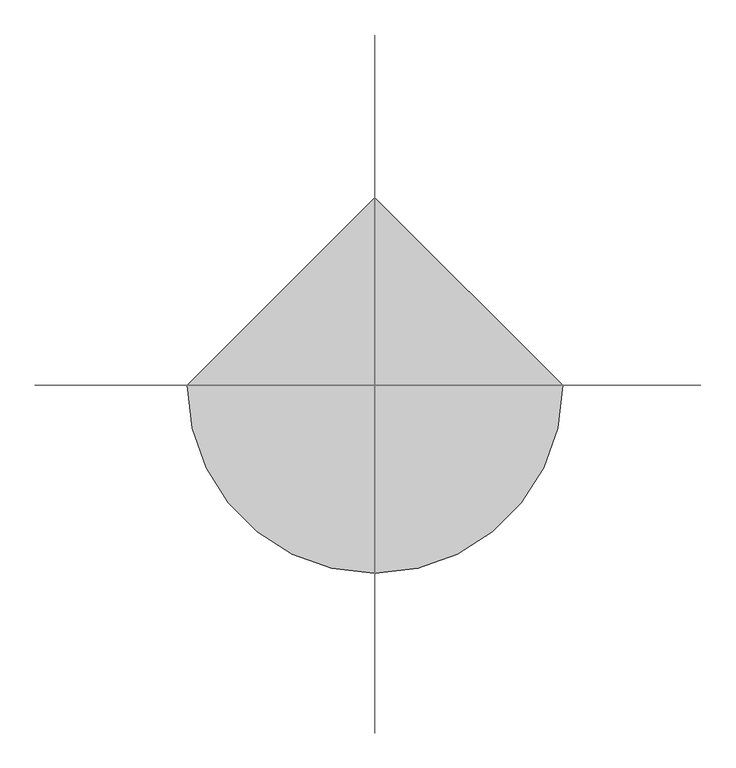
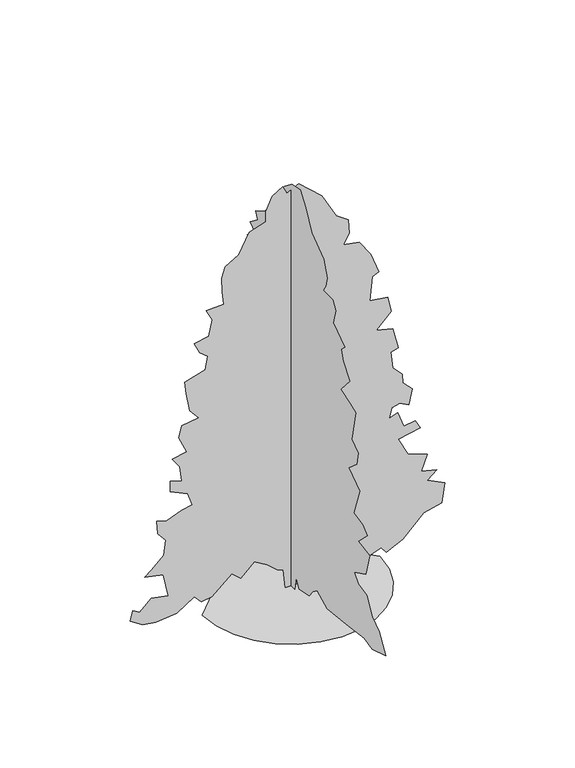
"""IFC4 building model written with IfcOpenShell, lengths in millimetres: proxy geometry, colorado spruce 26066 : colorado spruce 26066."""

import ifcopenshell
import ifcopenshell.guid

model = None  # the IFC model being written
_history = None  # IfcOwnerHistory: only IFC2X3 demands one
_inside = {}  # id of a spatial element -> (the spatial element, [elements in it])
_under = {}  # id of a project, library or spatial element -> (it, [spatial elements below it])
_declared = {}  # id of a project -> (the project, [libraries it declares])
_typed = {}  # id of a type object -> (the type object, [elements of that type])
_made_of = {}  # id of a material, layer set ... -> (it, [elements and type objects made of it])


def new_model(schema):
    """Start an empty IFC model of exactly this schema.

    Asked for "IFC4X3", IfcOpenShell would pick the latest addendum, in which some entities
    have other attributes; the version numbers below select the first issue.
    IFC2X3 requires an IfcOwnerHistory on every rooted entity: one is made here for all.
    """
    global model, _history
    if schema == "IFC4X3":
        model = ifcopenshell.file(schema_version=(4, 3, 0, 0))
    else:
        model = ifcopenshell.file(schema=schema)
    _inside.clear()
    _under.clear()
    _declared.clear()
    _typed.clear()
    _made_of.clear()
    _history = None
    if model.schema == "IFC2X3":
        org = make("IfcOrganization", Name="unknown")
        user = make(
            "IfcPersonAndOrganization",
            ThePerson=make("IfcPerson", FamilyName="unknown"),
            TheOrganization=org,
        )
        app = make(
            "IfcApplication",
            ApplicationDeveloper=org,
            Version="unknown",
            ApplicationFullName="unknown",
            ApplicationIdentifier="unknown",
        )
        _history = make(
            "IfcOwnerHistory",
            OwningUser=user,
            OwningApplication=app,
            ChangeAction="ADDED",
            CreationDate=0,
        )
    return model


def make(cls, **values):
    """One entity of the class cls with the attributes given. An attribute that is None is left unset."""
    return model.create_entity(
        cls, **{name: value for name, value in values.items() if value is not None}
    )


def rooted(cls, **values):
    """An entity with a GlobalId (a new one), such as an element, a storey or a relation."""
    return make(cls, GlobalId=ifcopenshell.guid.new(), OwnerHistory=_history, **values)


def si_unit(unit_type, name, prefix=None):
    """IfcSIUnit, for example si_unit("LENGTHUNIT", "METRE", prefix="MILLI")."""
    return make("IfcSIUnit", UnitType=unit_type, Prefix=prefix, Name=name)


def assignment(units):
    """IfcUnitAssignment: the units of a project."""
    return None if units is None else make("IfcUnitAssignment", Units=units)


def point(xyz):
    """IfcCartesianPoint."""
    return None if xyz is None else make("IfcCartesianPoint", Coordinates=xyz)


def direction(xyz):
    """IfcDirection."""
    return None if xyz is None else make("IfcDirection", DirectionRatios=xyz)


def frame(location, z_axis=None, x_axis=None):
    """IfcAxis2Placement3D, a coordinate frame: its origin and axes. An axis left out is left unset."""
    return make(
        "IfcAxis2Placement3D",
        Location=point(location),
        Axis=direction(z_axis),
        RefDirection=direction(x_axis),
    )


def origin():
    """The frame at (0, 0, 0) with its axes left unset."""
    return frame((0.0, 0.0, 0.0))


def place(relative_to, where):
    """IfcLocalPlacement: puts the frame where relative to a parent placement (None: the world)."""
    return make(
        "IfcLocalPlacement", PlacementRelTo=relative_to, RelativePlacement=where
    )


def context(
    kind, dimensions, precision=None, world=None, true_north=None, identifier=None
):
    """IfcGeometricRepresentationContext, for example the 3D "Model" context."""
    return make(
        "IfcGeometricRepresentationContext",
        ContextIdentifier=identifier,
        ContextType=kind,
        CoordinateSpaceDimension=dimensions,
        Precision=precision,
        WorldCoordinateSystem=world,
        TrueNorth=true_north,
    )


def project(units=None, contexts=None):
    """IfcProject with its units and contexts."""
    return rooted(
        "IfcProject",
        Name="project",
        RepresentationContexts=contexts,
        UnitsInContext=assignment(units),
    )


def spatial(cls, under=None, at=None, **own):
    """A site, building, storey or space (cls), placed at a placement, below another one or the project."""
    s = rooted(cls, ObjectPlacement=at, **own)
    if under is not None:
        _under.setdefault(under.id(), (under, []))[1].append(s)
    return s


def point_list(points):
    """IfcCartesianPointList2D or 3D."""
    cls = (
        "IfcCartesianPointList2D" if len(points[0]) == 2 else "IfcCartesianPointList3D"
    )
    return make(cls, CoordList=points)


def triangles(points, corners, closed=None, point_numbers=None):
    """IfcTriangulatedFaceSet: each triangle names its three corners, points numbered from 1."""
    return make(
        "IfcTriangulatedFaceSet",
        Coordinates=point_list(points),
        Closed=closed,
        CoordIndex=corners,
        PnIndex=point_numbers,
    )


def shape(context_of_items, identifier, shape_type, items):
    """IfcShapeRepresentation: the items that make up one representation, for example the "Body"."""
    return make(
        "IfcShapeRepresentation",
        ContextOfItems=context_of_items,
        RepresentationIdentifier=identifier,
        RepresentationType=shape_type,
        Items=items,
    )


def source(mapping_origin, context_of_items, identifier, shape_type, items):
    """IfcRepresentationMap: a shape defined once, which mapped items show again and again."""
    return make(
        "IfcRepresentationMap",
        MappingOrigin=mapping_origin,
        MappedRepresentation=shape(context_of_items, identifier, shape_type, items),
    )


def transform(
    local_origin,
    x_axis=None,
    y_axis=None,
    z_axis=None,
    scale=None,
    scale2=None,
    scale3=None,
    uniform=True,
):
    """IfcCartesianTransformationOperator3D, or its non-uniform kind. x_axis, y_axis, z_axis: its Axis1, 2, 3."""
    if uniform:
        return make(
            "IfcCartesianTransformationOperator3D",
            Axis1=direction(x_axis),
            Axis2=direction(y_axis),
            LocalOrigin=point(local_origin),
            Scale=scale,
            Axis3=direction(z_axis),
        )
    return make(
        "IfcCartesianTransformationOperator3DnonUniform",
        Axis1=direction(x_axis),
        Axis2=direction(y_axis),
        LocalOrigin=point(local_origin),
        Scale=scale,
        Axis3=direction(z_axis),
        Scale2=scale2,
        Scale3=scale3,
    )


def mapped(mapping_source, mapping_target):
    """IfcMappedItem: shows the shape of a source again, moved by a transform."""
    return make(
        "IfcMappedItem", MappingSource=mapping_source, MappingTarget=mapping_target
    )


def made_of(thing, what):
    """Note that an element or type object is made of a material, layer set ...; save() writes the relation."""
    if what is not None:
        _made_of.setdefault(what.id(), (what, []))[1].append(thing)
    return thing


def element(
    cls,
    number,
    at=None,
    inside=None,
    cuts=None,
    type_object=None,
    material=None,
    context=None,
    identifier="Body",
    shape_type=None,
    held_by="IfcProductDefinitionShape",
    body=None,
    shapes=None,
    **own,
):
    """One element of the class cls, such as IfcWall. Its Tag is "e" and its number.

    at: its placement. inside: the storey or other place that contains it. cuts: it is an
    opening in that element (IfcRelVoidsElement). A single representation is given by context,
    identifier, shape_type and body (its items); several are given by shapes. held_by: the class
    of the entity that holds the representations. save() writes the other relations.
    """
    e = rooted(cls, Tag="e%d" % number, ObjectPlacement=at, **own)
    if body is not None:
        shapes = [shape(context, identifier, shape_type, body)]
    if shapes is not None:
        e.Representation = make(held_by, Representations=shapes)
    if inside is not None:
        _inside.setdefault(inside.id(), (inside, []))[1].append(e)
    if cuts is not None:
        rooted(
            "IfcRelVoidsElement", RelatingBuildingElement=cuts, RelatedOpeningElement=e
        )
    if type_object is not None:
        _typed.setdefault(type_object.id(), (type_object, []))[1].append(e)
    return made_of(e, material)


def aggregate(whole, parts):
    """IfcRelAggregates: a whole, such as a stair, and the parts it consists of."""
    return rooted("IfcRelAggregates", RelatingObject=whole, RelatedObjects=parts)


def save(model, path):
    """Write the relations noted so far, then the file.

    IfcRelAggregates (storeys below a building ...), IfcRelContainedInSpatialStructure (elements
    in a storey), IfcRelDefinesByType, IfcRelAssociatesMaterial and IfcRelDeclares: one each for
    every whole, place, type object, material and project.
    """
    for whole, parts in _under.values():
        aggregate(whole, parts)
    for where, things in _inside.values():
        rooted(
            "IfcRelContainedInSpatialStructure",
            RelatedElements=things,
            RelatingStructure=where,
        )
    for kind, things in _typed.values():
        rooted("IfcRelDefinesByType", RelatedObjects=things, RelatingType=kind)
    for what, things in _made_of.values():
        rooted("IfcRelAssociatesMaterial", RelatedObjects=things, RelatingMaterial=what)
    for by, libraries in _declared.values():
        rooted("IfcRelDeclares", RelatingContext=by, RelatedDefinitions=libraries)
    model.write(path)


def entourage_51173285(model_context):
    return source(origin(), model_context, "Body", "Tessellation", [
        triangles([(2.3e-06, 50.6216921, 3.68e-05), (9.8e-06, 78.1276076, 213.1710181), (1.43e-05, 112.5100566, 309.4405598), (1.77e-05, 236.2865403, 240.6769336), (2.27e-05, 387.5684217, 178.7885601), (2.95e-05, 559.4807118, 151.2826536), (3.74e-05, 731.8705164, 158.5998759), (3.48e-05, 752.0228474, 41.258996), (4.28e-05, 875.7995945, 123.776738), (4.61e-05, 1007.1354006, 36.9163581), (5.13e-05, 1102.7231707, 68.7649115), (5.94e-05, 1288.3895267, 61.888369), (6.59e-05, 1377.7823261, 144.4061111), (8e-05, 1570.324498, 330.0704415), (7.64e-05, 1453.423494, 385.0817639), (7.29e-05, 1350.2767376, 419.465748), (6.83e-05, 1254.1961197, 411.4393484), (7.07e-05, 1233.3757336, 522.6126134), (7.48e-05, 1260.8813221, 618.883663), (8.24e-05, 1357.1524807, 728.9063078), (7.87e-05, 1260.8813221, 749.5362259), (8.41e-05, 1336.5226353, 818.3016506), (7.99e-05, 1219.624102, 852.6830549), (7.62e-05, 1095.8474276, 914.5726639), (7.72e-05, 1032.2102509, 1041.9130743), (8.57e-05, 1192.1185135, 1086.4849903), (9.06e-05, 1260.8813221, 1148.3720558), (8.72e-05, 1171.4885954, 1169.0019739), (8.31e-05, 1020.2061871, 1258.3973167), (8.97e-05, 1130.2288319, 1313.4086391), (9.55e-05, 1139.1290154, 1494.4927895), (9.04e-05, 1013.3279005, 1512.8265541), (8.63e-05, 903.3052557, 1540.3321426), (9.07e-05, 919.5358784, 1665.6252216), (9.79e-05, 1053.5310425, 1703.3976254), (0.0001031, 1082.0933252, 1836.0212162), (9.76e-05, 972.0706804, 1815.3912254), (9.84e-05, 902.5889477, 1949.2238995), (0.0001046, 978.9464235, 2042.3148743), (0.0001028, 882.6754103, 2124.8319305), (0.0001091, 978.9464235, 2193.5973553), (0.000112, 1006.4520847, 2248.6086777), (0.0001076, 834.539831, 2358.6337933), (0.0001087, 813.9099855, 2427.3966019), (0.0001169, 951.4407623, 2496.1621719), (0.0001168, 889.5511534, 2585.5674706), (0.0001125, 752.0228474, 2647.4418915), (0.0001196, 841.4156467, 2750.5914093), (0.0001179, 745.1445608, 2839.9740349), (0.0001151, 621.3703571, 2929.3819496), (0.0001181, 614.4919979, 3039.4147682), (0.0001241, 717.6388996, 3087.5475861), (0.0001224, 642.0002026, 3142.5639954), (0.000119, 552.6049324, 3163.1888992), (0.0001267, 669.5058638, 3245.688224), (0.000124, 545.729153, 3341.9794395), (0.0001276, 580.1105936, 3410.7374519), (0.0001236, 435.7039647, 3493.2617752), (0.000122, 318.802997, 3617.0361969), (0.0001233, 241.6693149, 3775.8113892), (0.000122, 98.7569716, 3947.1090729), (0.0001198, -11.2668813, 4036.4916985), (0.0001145, -148.7964954, 4063.9999031), (0.0001065, -245.067327, 3940.2257721), (9.64e-05, -341.337886, 3747.6936287), (8.32e-05, -540.7558373, 3603.2693047), (7.6e-05, -595.7671597, 3445.1289574), (7.44e-05, -568.2614985, 3348.8374512), (7.41e-05, -533.8800579, 3286.9630302), (6.73e-05, -685.1624662, 3286.9630302), (6.27e-05, -733.2979729, 3204.4384163), (6.03e-05, -692.0382093, 3060.0396721), (4.78e-05, -884.5803812, 2929.3819496), (4.89e-05, -822.6907722, 2874.3655403), (4.43e-05, -857.07472, 2771.2160225), (3.55e-05, -967.0973648, 2640.5585907), (3.71e-05, -815.8149565, 2468.6562927), (2.85e-05, -975.0983299, 2418.8978474), (2.34e-05, -1063.3684507, 2379.2636387), (1.71e-05, -1001.4787691, 2076.6963512), (1.03e-05, -1104.6282143, 2001.0551834), (7.5e-06, -1083.9982962, 1877.2784363), (9.8e-06, -953.3432625, 1760.3800484), (-1.8e-06, -1132.1338755, 1636.6033012), (-5.6e-06, -1028.9869738, 1354.6658592), (-1.32e-05, -1180.2693821, 1327.1601254), (-1.84e-05, -1255.9105499, 1265.2730598), (-1.62e-05, -1104.6282143, 1113.9906515), (-2.56e-05, -1297.16777, 1086.4849903), (-2.93e-05, -1228.4049614, 859.5588707), (-2.37e-05, -1042.7385326, 770.1660713), (-2.89e-05, -1104.6282143, 687.6490877), (-3.62e-05, -1249.032336, 660.1434265), (-4.49e-05, -1338.4276062, 501.9827316), (-5.26e-05, -1455.3284649, 419.465748), (-6.25e-05, -1558.4753666, 240.6769336), (-5.47e-05, -1338.4276062, 171.9120176), (-4.78e-05, -1203.4697828, 202.7582816), (-3.57e-05, -909.8228811, 166.6996904), (-2.27e-05, -595.7671597, 130.6530262), (-1.29e-05, -430.7306491, 213.1710181), (-1.15e-05, -361.9677678, 158.1589326), (-1.1e-05, -300.0781407, 82.5177376), (-4.6e-06, -135.0434104, 48.1355384), (1e-07, -87.2685559, 135.4498173), (-2.7e-06, -59.4022154, 3.35e-05), (-52.2236701, 1.3e-06, 3.68e-05), (-72.8530386, -2.11e-05, 185.6651025), (-127.8648697, -2.04e-05, 206.2944756), (-224.1356831, -2.12e-05, 288.8132396), (-347.9113947, -2.09e-05, 364.4544256), (-478.5664647, 3.3e-06, 240.6769336), (-561.0834483, 2.4e-06, 316.3188827), (-753.6255838, 1.55e-05, 151.2826536), (-850.3106707, 1.89e-05, 139.1823475), (-918.659551, 1.76e-05, 213.1710181), (-1083.6960617, 2.75e-05, 103.147365), (-1283.1139767, 4.91e-05, 82.5179919), (-1406.8907238, 5.18e-05, 103.147365), (-1523.7917278, 5.2e-05, 178.7885601), (-1503.1617371, 4.7e-05, 275.0591373), (-1434.3964577, 4.68e-05, 233.8003911), (-1324.3711967, 2.42e-05, 336.9487644), (-1166.2130453, 2.07e-05, 309.4405598), (-1212.8550385, 1.19e-05, 536.5622706), (-1386.2608784, 1.56e-05, 570.7481564), (-1324.3711967, 1.16e-05, 618.883663), (-1207.4728088, 3.2e-06, 728.9063078), (-1186.8428907, -3.9e-06, 873.312973), (-1262.4841312, -5.6e-06, 962.7082432), (-1276.2382336, -1.11e-05, 1093.3607334), (-1179.9671476, -1.27e-05, 1065.8550722), (-1035.5604824, -3.42e-05, 1120.8663946), (-939.2894691, -3.8e-05, 1141.4963127), (-980.5492327, -4.23e-05, 1265.2730598), (-1145.7305019, -4.09e-05, 1342.6363609), (-1145.5831272, -4.57e-05, 1450.9368725), (-1035.5604824, -4.74e-05, 1416.5553955), (-1054.1152365, -5.34e-05, 1562.7171135), (-1124.9558252, -5.58e-05, 1664.1088898), (-987.4249758, -6.12e-05, 1691.6146236), (-1063.0661436, -6.63e-05, 1856.6484455), (-1035.5604824, -7.2e-05, 1966.6737064), (-877.402331, -9.27e-05, 1994.179295), (-959.9193146, -9.46e-05, 2090.4504536), (-994.3007915, -0.0001019, 2276.1142662), (-1008.0548212, -0.0001067, 2393.0152702), (-815.512722, -0.0001152, 2454.9021904), (-788.0070608, -0.0001215, 2578.6841698), (-863.6482286, -0.000122, 2640.5585907), (-918.659551, -0.0001253, 2750.5914093), (-778.8249178, -0.0001453, 2774.1370651), (-746.7472973, -0.0001532, 2929.3819496), (-801.7586197, -0.0001565, 3039.4147682), (-636.7246525, -0.0001617, 3046.2727798), (-650.4762114, -0.0001671, 3176.9302116), (-657.3544979, -0.0001731, 3314.4712349), (-622.9705502, -0.0001787, 3417.6207527), (-495.5108156, -0.0002008, 3495.9796326), (-396.0469377, -0.0002122, 3685.7939186), (-237.8885137, -0.0002191, 3733.9270271), (-237.8885137, -0.0002237, 3837.0762543), (-176.0001583, -0.0002314, 3967.7339767), (-79.7295811, -0.000237, 4029.6083977), (-38.4705851, -0.0002349, 3953.9670845), (71.553068, -0.0002554, 4008.9834938), (291.5996066, -0.000253, 3809.5680496), (429.1304561, -0.0002313, 3562.0197876), (546.0314238, -0.0002458, 3479.4951736), (552.9072032, -0.0002251, 3341.9794395), (497.8958808, -0.0002192, 3245.688224), (649.1782528, -0.0002225, 3218.2053085), (759.2008976, -0.0002187, 3060.0396721), (834.8420654, -0.000212, 2860.6242279), (772.2870174, -0.0002087, 2828.0866791), (745.4493387, -0.0001977, 2599.3090736), (917.359049, -0.0002016, 2571.800869), (951.7430695, -0.0001958, 2420.5208588), (807.3364769, -0.0001854, 2282.9926254), (965.4946283, -0.0001882, 2241.7327892), (1020.5084942, -0.0001656, 2028.5607719), (944.8647102, -0.0001627, 2014.8092857), (965.4946283, -0.000156, 1849.7727024), (1056.4342083, -0.0001542, 1750.4358879), (1061.7657143, -0.0001505, 1664.1088898), (1151.1609844, -0.0001492, 1574.7136196), (1116.7770367, -0.0001414, 1423.4311386), (1034.2600531, -0.0001411, 1471.5667179), (958.6188126, -0.0001379, 1450.9368725), (931.1131514, -0.0001328, 1354.6658592), (1013.630135, -0.0001365, 1382.1714478), (1068.6414574, -0.0001311, 1224.0132236), (1178.6666456, -0.0001353, 1244.6432144), (1226.8021523, -0.0001327, 1155.2478716), (1020.5084942, -0.0001247, 1113.9906515), (1109.9012209, -0.0001046, 935.2000385), (1295.567577, -0.0001218, 866.4371572), (1236.1544884, -9.85e-05, 715.1572924), (1384.9603764, -0.0001014, 680.7708012), (1295.567577, -9.54e-05, 605.129597), (1460.6015442, -9.66e-05, 522.6126134), (1433.0959557, -8.72e-05, 330.0704415), (1261.1836292, -8.02e-05, 288.8132396), (1062.7105694, -6.57e-05, 95.753176), (903.6074902, -4.28e-05, 20.6293708), (855.4719835, -4.42e-05, 82.5177376), (674.9694111, -3.6e-05, 21.2873589), (484.1417785, -3e-05, 13.7529317), (408.5005743, -3.08e-05, 82.5177376), (236.5885567, -2.85e-05, 144.4061111), (74.3397029, -2.22e-05, 111.1694498), (57.799983, -1.67e-05, 3.35e-05), (-841.6823456, -4.7e-06, 6.03e-05), (-819.4294161, -192.8576323, 5.39e-05), (-756.0589382, -369.9662258, 4.68e-05), (-656.640806, -526.2524348, 3.91e-05), (-526.2524348, -656.640806, 3.14e-05), (-369.9662258, -756.0589382, 2.37e-05), (-192.8576323, -819.4294161, 1.66e-05), (3.68e-05, -841.6823456, 1.02e-05), (192.8576323, -819.4294161, 5.1e-06), (369.9662258, -756.0589382, 1.7e-06), (526.2524348, -656.640806, 0.0), (656.640806, -526.2524348, 0.0), (756.0589382, -369.9662258, 1.7e-06), (819.4294161, -192.8576323, 5.1e-06), (841.6823456, 7.8e-05, 1.02e-05), (-0.0001104, 841.6823456, 6.03e-05)], [[26, 27, 28], [21, 22, 23], [19, 20, 21], [51, 52, 53], [7, 8, 9], [35, 36, 37], [13, 14, 15], [34, 35, 37], [54, 55, 56], [72, 73, 74], [95, 96, 97], [88, 89, 90], [44, 45, 46], [86, 87, 88], [85, 86, 88], [51, 53, 54], [44, 46, 47], [88, 90, 91], [13, 15, 16], [13, 16, 17], [38, 39, 40], [25, 26, 28], [25, 28, 29], [47, 48, 49], [56, 57, 58], [30, 31, 32], [29, 30, 32], [41, 42, 43], [40, 41, 43], [106, 1, 2], [105, 106, 2], [75, 76, 77], [94, 95, 97], [94, 97, 98], [78, 79, 80], [83, 84, 85], [29, 32, 33], [103, 104, 105], [12, 13, 17], [11, 12, 17], [77, 78, 80], [102, 103, 105], [62, 63, 64], [80, 81, 82], [80, 82, 83], [61, 62, 64], [61, 64, 65], [60, 61, 65], [59, 60, 65], [69, 70, 71], [69, 71, 72], [94, 98, 99], [93, 94, 99], [92, 93, 99], [92, 99, 100], [91, 92, 100], [91, 100, 101], [47, 49, 50], [9, 10, 11], [9, 11, 17], [9, 17, 18], [7, 9, 18], [59, 65, 66], [59, 66, 67], [59, 67, 68], [59, 68, 69], [58, 59, 69], [56, 58, 69], [54, 56, 69], [54, 69, 72], [51, 54, 72], [50, 51, 72], [50, 72, 74], [50, 74, 75], [50, 75, 77], [47, 50, 77], [44, 47, 77], [43, 44, 77], [40, 43, 77], [40, 77, 80], [40, 80, 83], [38, 40, 83], [38, 83, 85], [37, 38, 85], [34, 37, 85], [33, 34, 85], [29, 33, 85], [25, 29, 85], [25, 85, 88], [25, 88, 91], [25, 91, 101], [25, 101, 102], [24, 25, 102], [23, 24, 102], [21, 23, 102], [105, 2, 3], [102, 105, 3], [21, 102, 3], [21, 3, 4], [21, 4, 5], [21, 5, 6], [21, 6, 7], [21, 7, 18], [19, 21, 18], [125, 126, 127], [198, 199, 200], [153, 154, 155], [139, 140, 141], [130, 131, 132], [120, 121, 122], [119, 120, 122], [186, 187, 188], [136, 137, 138], [135, 136, 138], [150, 151, 152], [193, 194, 195], [192, 193, 195], [125, 127, 128], [180, 181, 182], [163, 164, 165], [185, 186, 188], [196, 197, 198], [190, 191, 192], [111, 112, 113], [212, 107, 108], [211, 212, 108], [173, 174, 175], [149, 150, 152], [179, 180, 182], [129, 130, 132], [146, 147, 148], [204, 205, 206], [200, 201, 202], [200, 202, 203], [162, 163, 165], [190, 192, 195], [165, 166, 167], [118, 119, 122], [118, 122, 123], [118, 123, 124], [117, 118, 124], [116, 117, 124], [176, 177, 178], [176, 178, 179], [129, 132, 133], [185, 188, 189], [142, 143, 144], [141, 142, 144], [161, 162, 165], [161, 165, 167], [161, 167, 168], [116, 124, 125], [145, 146, 148], [144, 145, 148], [114, 115, 116], [113, 114, 116], [113, 116, 125], [113, 125, 128], [113, 128, 129], [113, 129, 133], [113, 133, 134], [111, 113, 134], [168, 169, 170], [168, 170, 171], [161, 168, 171], [160, 161, 171], [159, 160, 171], [158, 159, 171], [157, 158, 171], [156, 157, 171], [155, 156, 171], [171, 172, 173], [171, 173, 175], [155, 171, 175], [155, 175, 176], [153, 155, 176], [152, 153, 176], [149, 152, 176], [149, 176, 179], [148, 149, 179], [144, 148, 179], [144, 179, 182], [144, 182, 183], [141, 144, 183], [139, 141, 183], [138, 139, 183], [135, 138, 183], [134, 135, 183], [111, 134, 183], [110, 111, 183], [110, 183, 184], [110, 184, 185], [110, 185, 189], [110, 189, 190], [110, 190, 195], [109, 110, 195], [108, 109, 195], [211, 108, 195], [210, 211, 195], [210, 195, 196], [209, 210, 196], [209, 196, 198], [208, 209, 198], [207, 208, 198], [206, 207, 198], [204, 206, 198], [203, 204, 198], [200, 203, 198], [227, 228, 213], [226, 227, 213], [226, 213, 214], [225, 226, 214], [225, 214, 215], [225, 215, 216], [224, 225, 216], [223, 224, 216], [223, 216, 217], [223, 217, 218], [223, 218, 219], [223, 219, 220], [223, 220, 221], [223, 221, 222]], closed=False),
    ])


if __name__ == "__main__":
    model = new_model("IFC4")
    model_context = context("Model", 3, world=origin())
    ifc_project = project(units=[si_unit("LENGTHUNIT", "METRE", prefix="MILLI")], contexts=[model_context])
    site = spatial("IfcSite", under=ifc_project)
    building = spatial("IfcBuilding", under=site)
    placement = place(None, origin())
    entourage_shape = entourage_51173285(model_context)
    element("IfcBuildingElementProxy", 1, Name="colorado spruce 26066 : colorado spruce 26066", ObjectType="colorado spruce 26066 : colorado spruce 26066", at=placement, inside=building, context=model_context, shape_type="MappedRepresentation", body=[
        mapped(entourage_shape, transform((0.0, 0.0, 0.0), x_axis=(1.0, 0.0, 0.0), y_axis=(0.0, 1.0, 0.0), z_axis=(0.0, 0.0, 1.0))),
    ])
    save(model, "model.ifc")

# Revit data of these elements
# Type "colorado spruce 26066 : colorado spruce 26066"
#   built-in parameter 1005195 = "RPC-16-G0M4-N9PX-U6TN-C000-ST1L-LVER-AU"
#   Height = 0
